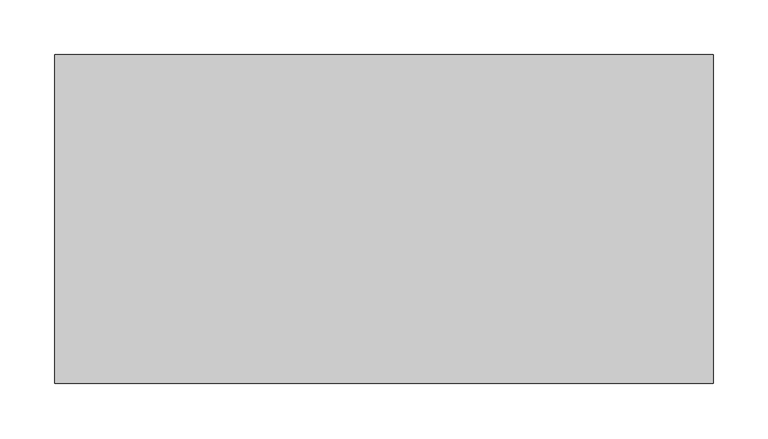
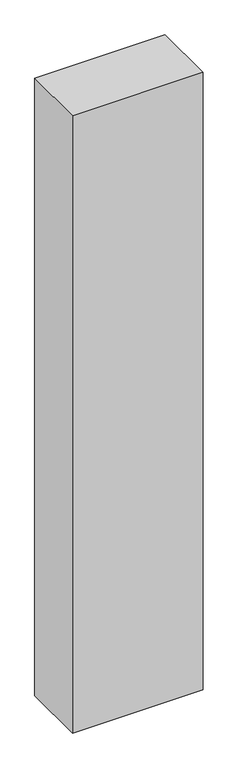
"""IFC4 building model written with IfcOpenShell, lengths in millimetres: column geometry, 5dki STB-Stützen rechteckig : 5dki Stütze recht. 60x30 cm C35/45."""

from ifc_helpers import new_model, si_unit, frame, origin, place, context, project, spatial, polyline, outline, extrude, source, transform, mapped, element, save


def column_b848c13c(model_context):
    return source(origin(), model_context, "Body", "SweptSolid", [
        extrude(outline(polyline([(300.0, 150.0), (300.0, -150.0), (-300.0, -150.0), (-300.0, 150.0), (300.0, 150.0)])), frame((0.0, 0.0, -4200.0), z_axis=(0.0, 0.0, 1.0), x_axis=(1.0, 0.0, 0.0)), (0.0, 0.0, 1.0), 3000.0),
    ])


if __name__ == "__main__":
    model = new_model("IFC4")
    model_context = context("Model", 3, world=origin())
    ifc_project = project(units=[si_unit("LENGTHUNIT", "METRE", prefix="MILLI")], contexts=[model_context])
    site = spatial("IfcSite", under=ifc_project)
    building = spatial("IfcBuilding", under=site)
    placement = place(None, origin())
    column_shape = column_b848c13c(model_context)
    element("IfcColumn", 1, ObjectType="5dki STB-Stützen rechteckig : 5dki Stütze recht. 60x30 cm C35/45", at=placement, inside=building, context=model_context, shape_type="MappedRepresentation", body=[
        mapped(column_shape, transform((0.0, 0.0, 0.0), x_axis=(1.0, 0.0, 0.0), y_axis=(0.0, 1.0, 0.0), z_axis=(0.0, 0.0, 1.0))),
    ])
    save(model, "model.ifc")

# Revit data of these elements
# Type "5dki STB-Stützen rechteckig : 5dki Stütze recht. 60x30 cm C35/45"
#   cpiFitMatchKey = "5D-KI-STB-OB-ST-REC"
#   cpiComponentType = "Column"
#   5d Materialgüte = "C35/45"
#   Tiefe = 0.300 m
#   Breite = 0.600 m
#   5dki Bewehrung Stab kg pro m3 = 0
#   5dki Sichtbeton SB3/SB4 [instance default] = no
#   Structural Material = 5d Beton - Stahlbeton
#   Assembly Code = ""
# Element 1 (IfcColumn, "5dki STB-Stützen rechteckig : 5dki Stütze recht. 60x30 cm C35/45")
#   Materials on its faces: "5d Beton - Stahlbeton"
# Materials
#   "5d Beton - Stahlbeton": class "5dki", colour RGB 200 200 200, transparency 0, Cost = 0
